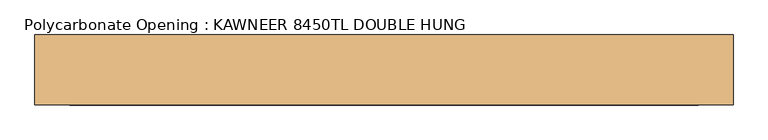
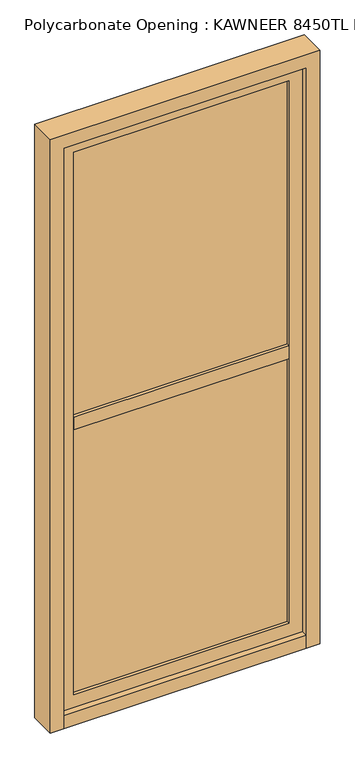
"""IFC4 building model written with IfcOpenShell, lengths in millimetres: door geometry, Polycarbonate Opening : KAWNEER 8450TL DOUBLE HUNG."""

from ifc_helpers import new_model, si_unit, frame, origin, origin_with_axes, place, context, project, spatial, polyline, outline, extrude, source, transform, mapped, element, save


def polycarbonate_opening_kawneer_8450tl_double_hung_4e587098(model_context):
    return source(origin(), model_context, "Body", "SweptSolid", [
        extrude(outline(polyline([(457.2, 0.0), (457.2, -25.4), (-457.2, -25.4), (-457.2, 0.0), (457.2, 0.0)])), frame((0.0, 0.0, 50.8), z_axis=(0.0, 0.0, 1.0), x_axis=(1.0, 0.0, 0.0)), (0.0, 0.0, 1.0), 2260.6),
        extrude(outline(polyline([(2311.4, -457.2), (0.0, -457.2), (0.0, 457.2), (2311.4, 457.2), (2311.4, -457.2)]), holes=[polyline([(101.6, 406.4), (101.6, -406.4), (2260.6, -406.4), (2260.6, 406.4), (101.6, 406.4)])]), frame((0.0, -38.1, 0.0), z_axis=(0.0, 1.0, 0.0), x_axis=(0.0, 0.0, 1.0)), (0.0, 0.0, 1.0), 50.8),
        extrude(outline(polyline([(2362.2, 508.0), (2362.2, -508.0), (0.0, -508.0), (0.0, -457.2), (2311.4, -457.2), (2311.4, 457.2), (0.0, 457.2), (0.0, 508.0), (2362.2, 508.0)])), frame((0.0, -63.5, 0.0), z_axis=(0.0, 1.0, 0.0), x_axis=(0.0, 0.0, 1.0)), (0.0, 0.0, 1.0), 101.6),
        extrude(outline(polyline([(406.4, 12.7), (406.4, -38.1), (-406.4, -38.1), (-406.4, 12.7), (406.4, 12.7)])), frame((0.0, 0.0, 1155.7), z_axis=(0.0, 0.0, 1.0), x_axis=(1.0, 0.0, 0.0)), (0.0, 0.0, 1.0), 50.8),
        extrude(outline(polyline([(457.2, 38.1), (457.2, -63.5), (-457.2, -63.5), (-457.2, 38.1), (457.2, 38.1)])), origin_with_axes(), (0.0, 0.0, 1.0), 50.8),
    ])


if __name__ == "__main__":
    model = new_model("IFC4")
    model_context = context("Model", 3, world=origin())
    ifc_project = project(units=[si_unit("LENGTHUNIT", "METRE", prefix="MILLI")], contexts=[model_context])
    site = spatial("IfcSite", under=ifc_project)
    building = spatial("IfcBuilding", under=site)
    placement = place(None, origin())
    polycarbonate_opening_kawneer_8450tl_double_hung_shape = polycarbonate_opening_kawneer_8450tl_double_hung_4e587098(model_context)
    element("IfcDoor", 1, ObjectType="Polycarbonate Opening : KAWNEER 8450TL DOUBLE HUNG", at=placement, inside=building, context=model_context, shape_type="MappedRepresentation", body=[
        mapped(polycarbonate_opening_kawneer_8450tl_double_hung_shape, transform((0.0, 0.0, 0.0), x_axis=(1.0, 0.0, 0.0), y_axis=(0.0, 1.0, 0.0), z_axis=(0.0, 0.0, 1.0))),
    ])
    save(model, "model.ifc")

# Revit data of these elements
# Type "Polycarbonate Opening : KAWNEER 8450TL DOUBLE HUNG"
#   Type Mark = "59"
#   OD_DS_Door_Material = "ALUM./GLAZING"
#   OD_DS_Door_Type = "STOREFRONT - SINGLE HUNG WINDOW"
#   OD_DS_Lockset = "-"
#   Analytic Construction = "<None>"
#   offset [instance default] = 0' - 2"
#   Stile = 0' - 2"
#   Mullion Width = 0' - 2"
#   Mullion Depth = 0' - 4"
#   Opening Size [instance default] = 5' - 1.50212"
#   Door Width [instance default] = 5' - 1.50212"
#   Window ON/OFF = no
#   Door On/Off = yes
#   Mullion Material = KAWNEER 8450TL DOUBLE HUNG (CLEAR ANODIZED ALUM) - TEMPERED INSULATED GLAZING (CARDINAL GLASS LoĒ²-240\nOR EQUIVALENT)
#   Glass Material = TEMPERED INSULATED GLAZING (CARDINAL GLASS LoĒ²-240\nOR EQUIVALENT)
#   Door Material = KAWNEER 8450TL DOUBLE HUNG (CLEAR ANODIZED ALUM) - TEMPERED INSULATED GLAZING (CARDINAL GLASS LoĒ²-240\nOR EQUIVALENT)
# Element 1 (IfcDoor, "Polycarbonate Opening : KAWNEER 8450TL DOUBLE HUNG")
#   offset = 0' - 0 1/2"
#   Materials on its faces: "KAWNEER 8450TL DOUBLE HUNG (CLEAR ANODIZED ALUM) - TEMPERED INSULATED GLAZING (CARDINAL GLASS LoĒ²-240\nOR EQUIVALENT)", "TEMPERED INSULATED GLAZING (CARDINAL GLASS LoĒ²-240\nOR EQUIVALENT)"
# Materials
#   "KAWNEER 8450TL DOUBLE HUNG (CLEAR ANODIZED ALUM) - TEMPERED INSULATED GLAZING (CARDINAL GLASS LoĒ²-240\nOR EQUIVALENT)": class "Metal", colour RGB 244 244 244, transparency 0, Description = "Aluminum 6061", Cost = 0
#   "TEMPERED INSULATED GLAZING (CARDINAL GLASS LoĒ²-240\nOR EQUIVALENT)": class "Glass", colour RGB 196 205 210, transparency 0.85, Description = "Soda Lime Glass", Cost = 0
